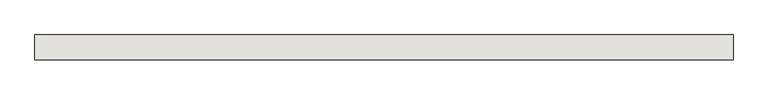
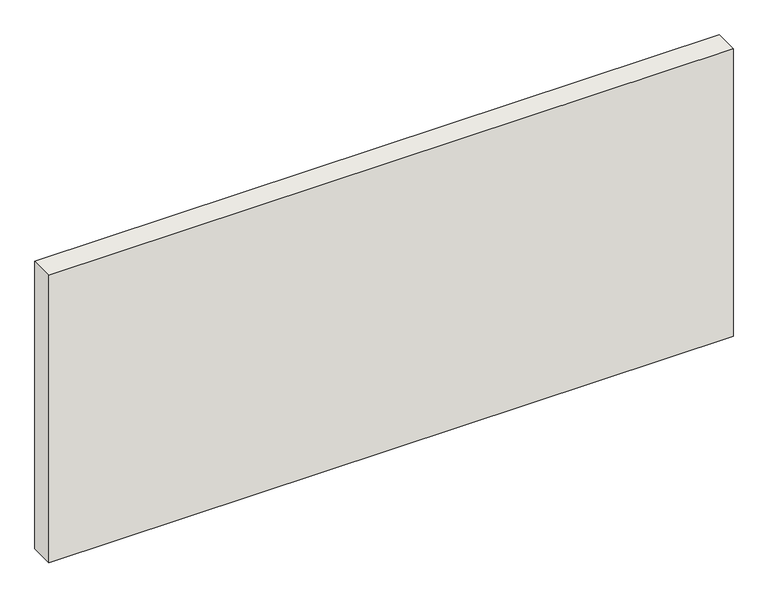
"""IFC4 building model written with IfcOpenShell, lengths in millimetres: wall geometry, Holzwand."""

import ifcopenshell
import ifcopenshell.guid

model = None  # the IFC model being written
_history = None  # IfcOwnerHistory: only IFC2X3 demands one
_inside = {}  # id of a spatial element -> (the spatial element, [elements in it])
_under = {}  # id of a project, library or spatial element -> (it, [spatial elements below it])
_declared = {}  # id of a project -> (the project, [libraries it declares])
_typed = {}  # id of a type object -> (the type object, [elements of that type])
_made_of = {}  # id of a material, layer set ... -> (it, [elements and type objects made of it])


def new_model(schema):
    """Start an empty IFC model of exactly this schema.

    Asked for "IFC4X3", IfcOpenShell would pick the latest addendum, in which some entities
    have other attributes; the version numbers below select the first issue.
    IFC2X3 requires an IfcOwnerHistory on every rooted entity: one is made here for all.
    """
    global model, _history
    if schema == "IFC4X3":
        model = ifcopenshell.file(schema_version=(4, 3, 0, 0))
    else:
        model = ifcopenshell.file(schema=schema)
    _inside.clear()
    _under.clear()
    _declared.clear()
    _typed.clear()
    _made_of.clear()
    _history = None
    if model.schema == "IFC2X3":
        org = make("IfcOrganization", Name="unknown")
        user = make(
            "IfcPersonAndOrganization",
            ThePerson=make("IfcPerson", FamilyName="unknown"),
            TheOrganization=org,
        )
        app = make(
            "IfcApplication",
            ApplicationDeveloper=org,
            Version="unknown",
            ApplicationFullName="unknown",
            ApplicationIdentifier="unknown",
        )
        _history = make(
            "IfcOwnerHistory",
            OwningUser=user,
            OwningApplication=app,
            ChangeAction="ADDED",
            CreationDate=0,
        )
    return model


def make(cls, **values):
    """One entity of the class cls with the attributes given. An attribute that is None is left unset."""
    return model.create_entity(
        cls, **{name: value for name, value in values.items() if value is not None}
    )


def rooted(cls, **values):
    """An entity with a GlobalId (a new one), such as an element, a storey or a relation."""
    return make(cls, GlobalId=ifcopenshell.guid.new(), OwnerHistory=_history, **values)


def si_unit(unit_type, name, prefix=None):
    """IfcSIUnit, for example si_unit("LENGTHUNIT", "METRE", prefix="MILLI")."""
    return make("IfcSIUnit", UnitType=unit_type, Prefix=prefix, Name=name)


def assignment(units):
    """IfcUnitAssignment: the units of a project."""
    return None if units is None else make("IfcUnitAssignment", Units=units)


def point(xyz):
    """IfcCartesianPoint."""
    return None if xyz is None else make("IfcCartesianPoint", Coordinates=xyz)


def direction(xyz):
    """IfcDirection."""
    return None if xyz is None else make("IfcDirection", DirectionRatios=xyz)


def frame(location, z_axis=None, x_axis=None):
    """IfcAxis2Placement3D, a coordinate frame: its origin and axes. An axis left out is left unset."""
    return make(
        "IfcAxis2Placement3D",
        Location=point(location),
        Axis=direction(z_axis),
        RefDirection=direction(x_axis),
    )


def origin():
    """The frame at (0, 0, 0) with its axes left unset."""
    return frame((0.0, 0.0, 0.0))


def origin_with_axes():
    """The frame at (0, 0, 0) with the z axis (0, 0, 1) and the x axis (1, 0, 0) written out."""
    return frame((0.0, 0.0, 0.0), z_axis=(0.0, 0.0, 1.0), x_axis=(1.0, 0.0, 0.0))


def place(relative_to, where):
    """IfcLocalPlacement: puts the frame where relative to a parent placement (None: the world)."""
    return make(
        "IfcLocalPlacement", PlacementRelTo=relative_to, RelativePlacement=where
    )


def context(
    kind, dimensions, precision=None, world=None, true_north=None, identifier=None
):
    """IfcGeometricRepresentationContext, for example the 3D "Model" context."""
    return make(
        "IfcGeometricRepresentationContext",
        ContextIdentifier=identifier,
        ContextType=kind,
        CoordinateSpaceDimension=dimensions,
        Precision=precision,
        WorldCoordinateSystem=world,
        TrueNorth=true_north,
    )


def project(units=None, contexts=None):
    """IfcProject with its units and contexts."""
    return rooted(
        "IfcProject",
        Name="project",
        RepresentationContexts=contexts,
        UnitsInContext=assignment(units),
    )


def spatial(cls, under=None, at=None, **own):
    """A site, building, storey or space (cls), placed at a placement, below another one or the project."""
    s = rooted(cls, ObjectPlacement=at, **own)
    if under is not None:
        _under.setdefault(under.id(), (under, []))[1].append(s)
    return s


def polyline(points):
    """IfcPolyline through the points."""
    return make("IfcPolyline", Points=[point(p) for p in points])


def outline(outer, holes=None, kind="AREA"):
    """IfcArbitraryClosedProfileDef: a profile drawn as a closed curve; with holes, ...WithVoids."""
    if holes is None:
        return make("IfcArbitraryClosedProfileDef", ProfileType=kind, OuterCurve=outer)
    return make(
        "IfcArbitraryProfileDefWithVoids",
        ProfileType=kind,
        OuterCurve=outer,
        InnerCurves=holes,
    )


def extrude(swept, where, along, depth):
    """IfcExtrudedAreaSolid: the profile swept, set in the frame where, extruded along a direction by depth."""
    return make(
        "IfcExtrudedAreaSolid",
        SweptArea=swept,
        Position=where,
        ExtrudedDirection=direction(along),
        Depth=depth,
    )


def shape(context_of_items, identifier, shape_type, items):
    """IfcShapeRepresentation: the items that make up one representation, for example the "Body"."""
    return make(
        "IfcShapeRepresentation",
        ContextOfItems=context_of_items,
        RepresentationIdentifier=identifier,
        RepresentationType=shape_type,
        Items=items,
    )


def source(mapping_origin, context_of_items, identifier, shape_type, items):
    """IfcRepresentationMap: a shape defined once, which mapped items show again and again."""
    return make(
        "IfcRepresentationMap",
        MappingOrigin=mapping_origin,
        MappedRepresentation=shape(context_of_items, identifier, shape_type, items),
    )


def transform(
    local_origin,
    x_axis=None,
    y_axis=None,
    z_axis=None,
    scale=None,
    scale2=None,
    scale3=None,
    uniform=True,
):
    """IfcCartesianTransformationOperator3D, or its non-uniform kind. x_axis, y_axis, z_axis: its Axis1, 2, 3."""
    if uniform:
        return make(
            "IfcCartesianTransformationOperator3D",
            Axis1=direction(x_axis),
            Axis2=direction(y_axis),
            LocalOrigin=point(local_origin),
            Scale=scale,
            Axis3=direction(z_axis),
        )
    return make(
        "IfcCartesianTransformationOperator3DnonUniform",
        Axis1=direction(x_axis),
        Axis2=direction(y_axis),
        LocalOrigin=point(local_origin),
        Scale=scale,
        Axis3=direction(z_axis),
        Scale2=scale2,
        Scale3=scale3,
    )


def mapped(mapping_source, mapping_target):
    """IfcMappedItem: shows the shape of a source again, moved by a transform."""
    return make(
        "IfcMappedItem", MappingSource=mapping_source, MappingTarget=mapping_target
    )


def made_of(thing, what):
    """Note that an element or type object is made of a material, layer set ...; save() writes the relation."""
    if what is not None:
        _made_of.setdefault(what.id(), (what, []))[1].append(thing)
    return thing


def element(
    cls,
    number,
    at=None,
    inside=None,
    cuts=None,
    type_object=None,
    material=None,
    context=None,
    identifier="Body",
    shape_type=None,
    held_by="IfcProductDefinitionShape",
    body=None,
    shapes=None,
    **own,
):
    """One element of the class cls, such as IfcWall. Its Tag is "e" and its number.

    at: its placement. inside: the storey or other place that contains it. cuts: it is an
    opening in that element (IfcRelVoidsElement). A single representation is given by context,
    identifier, shape_type and body (its items); several are given by shapes. held_by: the class
    of the entity that holds the representations. save() writes the other relations.
    """
    e = rooted(cls, Tag="e%d" % number, ObjectPlacement=at, **own)
    if body is not None:
        shapes = [shape(context, identifier, shape_type, body)]
    if shapes is not None:
        e.Representation = make(held_by, Representations=shapes)
    if inside is not None:
        _inside.setdefault(inside.id(), (inside, []))[1].append(e)
    if cuts is not None:
        rooted(
            "IfcRelVoidsElement", RelatingBuildingElement=cuts, RelatedOpeningElement=e
        )
    if type_object is not None:
        _typed.setdefault(type_object.id(), (type_object, []))[1].append(e)
    return made_of(e, material)


def aggregate(whole, parts):
    """IfcRelAggregates: a whole, such as a stair, and the parts it consists of."""
    return rooted("IfcRelAggregates", RelatingObject=whole, RelatedObjects=parts)


def save(model, path):
    """Write the relations noted so far, then the file.

    IfcRelAggregates (storeys below a building ...), IfcRelContainedInSpatialStructure (elements
    in a storey), IfcRelDefinesByType, IfcRelAssociatesMaterial and IfcRelDeclares: one each for
    every whole, place, type object, material and project.
    """
    for whole, parts in _under.values():
        aggregate(whole, parts)
    for where, things in _inside.values():
        rooted(
            "IfcRelContainedInSpatialStructure",
            RelatedElements=things,
            RelatingStructure=where,
        )
    for kind, things in _typed.values():
        rooted("IfcRelDefinesByType", RelatedObjects=things, RelatingType=kind)
    for what, things in _made_of.values():
        rooted("IfcRelAssociatesMaterial", RelatedObjects=things, RelatingMaterial=what)
    for by, libraries in _declared.values():
        rooted("IfcRelDeclares", RelatingContext=by, RelatedDefinitions=libraries)
    model.write(path)


def wall_fe2e87f2(model_context):
    return source(origin(), model_context, "Body", "SweptSolid", [
        extrude(outline(polyline([(0.0, 200.0), (5650.0, 200.0), (5650.0, 0.0), (0.0, 0.0), (0.0, 200.0)])), origin_with_axes(), (0.0, 0.0, 1.0), 2510.0),
    ])


if __name__ == "__main__":
    model = new_model("IFC4")
    model_context = context("Model", 3, world=origin())
    ifc_project = project(units=[si_unit("LENGTHUNIT", "METRE", prefix="MILLI")], contexts=[model_context])
    site = spatial("IfcSite", under=ifc_project)
    building = spatial("IfcBuilding", under=site)
    placement = place(None, origin())
    wall_shape = wall_fe2e87f2(model_context)
    element("IfcWall", 1, ObjectType="Holzwand", at=placement, inside=building, context=model_context, shape_type="MappedRepresentation", body=[
        mapped(wall_shape, transform((0.0, 0.0, 0.0), x_axis=(1.0, 0.0, 0.0), y_axis=(0.0, 1.0, 0.0), z_axis=(0.0, 0.0, 1.0))),
    ])
    save(model, "model.ifc")

# Revit data of these elements
# Element 1 (IfcWall, "Holzwand")
#   Materials on its faces: "holzschalung"
# Materials
#   "holzschalung": class "Unassigned", colour RGB 128 128 128, transparency 0
